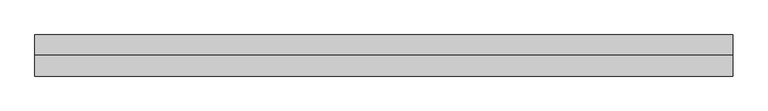
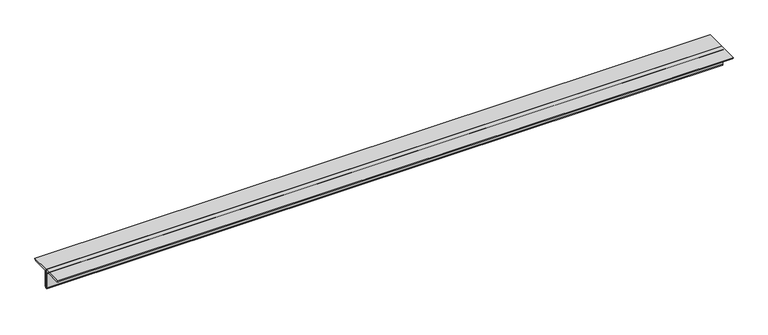
"""IFC4 building model written with IfcOpenShell, lengths in millimetres: member geometry, 0123_Steel Framing_2Ls-KSD3502 : H_SB_AR_S03_2Ls-130x130x12_HBR1."""

from ifc_helpers import new_model, si_unit, point, frame, frame_2d, origin, place, context, project, spatial, polyline, circle_curve, trimmed, segment, composite_curve, outline, extrude, source, transform, mapped, element, save


def member_7318b5d7(model_context):
    return source(origin(), model_context, "Body", "SweptSolid", [
        extrude(outline(composite_curve([segment(polyline([(0.0, 36.4), (0.0, -93.6)]), True, "CONTINUOUS"), segment(trimmed(circle_curve(frame_2d((0.0, -81.6)), 12.0), [point((0.0, -93.6))], [point((-12.0, -81.6))], False, "CARTESIAN"), True, "CONTINUOUS"), segment(polyline([(-12.0, -81.6), (-12.0, 12.4)]), True, "CONTINUOUS"), segment(trimmed(circle_curve(frame_2d((-24.0, 12.4)), 12.0), [point((-12.0, 12.4))], [point((-24.0, 24.4))], True, "CARTESIAN"), True, "CONTINUOUS"), segment(polyline([(-24.0, 24.4), (-118.0, 24.4)]), True, "CONTINUOUS"), segment(trimmed(circle_curve(frame_2d((-118.0, 36.4)), 12.0), [point((-118.0, 24.4))], [point((-130.0, 36.4))], False, "CARTESIAN"), True, "CONTINUOUS"), segment(polyline([(-130.0, 36.4), (0.0, 36.4)]), True, "CONTINUOUS")], self_intersect=False)), frame((-2254.4342987, 0.0, 0.0), z_axis=(1.0, 0.0, 0.0), x_axis=(0.0, 1.0, 0.0)), (0.0, 0.0, 1.0), 4412.2019305),
        extrude(outline(composite_curve([segment(polyline([(0.0, 36.4), (130.0, 36.4)]), True, "CONTINUOUS"), segment(trimmed(circle_curve(frame_2d((118.0, 36.4)), 12.0), [point((130.0, 36.4))], [point((118.0, 24.4))], False, "CARTESIAN"), True, "CONTINUOUS"), segment(polyline([(118.0, 24.4), (24.0, 24.4)]), True, "CONTINUOUS"), segment(trimmed(circle_curve(frame_2d((24.0, 12.4)), 12.0), [point((24.0, 24.4))], [point((12.0, 12.4))], True, "CARTESIAN"), True, "CONTINUOUS"), segment(polyline([(12.0, 12.4), (12.0, -81.6)]), True, "CONTINUOUS"), segment(trimmed(circle_curve(frame_2d((0.0, -81.6)), 12.0), [point((12.0, -81.6))], [point((0.0, -93.6))], False, "CARTESIAN"), True, "CONTINUOUS"), segment(polyline([(0.0, -93.6), (0.0, 36.4)]), True, "CONTINUOUS")], self_intersect=False)), frame((-2254.4342987, 0.0, 0.0), z_axis=(1.0, 0.0, 0.0), x_axis=(0.0, 1.0, 0.0)), (0.0, 0.0, 1.0), 4412.2019305),
    ])


if __name__ == "__main__":
    model = new_model("IFC4")
    model_context = context("Model", 3, world=origin())
    ifc_project = project(units=[si_unit("LENGTHUNIT", "METRE", prefix="MILLI")], contexts=[model_context])
    site = spatial("IfcSite", under=ifc_project)
    building = spatial("IfcBuilding", under=site)
    placement = place(None, origin())
    member_shape = member_7318b5d7(model_context)
    element("IfcMember", 1, ObjectType="0123_Steel Framing_2Ls-KSD3502 : H_SB_AR_S03_2Ls-130x130x12_HBR1", at=placement, inside=building, context=model_context, shape_type="MappedRepresentation", body=[
        mapped(member_shape, transform((0.0, 0.0, 0.0), x_axis=(1.0, 0.0, 0.0), y_axis=(0.0, 1.0, 0.0), z_axis=(0.0, 0.0, 1.0))),
    ])
    save(model, "model.ifc")

# Revit data of these elements
# Type "0123_Steel Framing_2Ls-KSD3502 : H_SB_AR_S03_2Ls-130x130x12_HBR1"
#   Type Mark = "HBR1"
#   Assembly Code = "B10"
#   Legs = "SLBB"
#   W = 8.97
#   Perimeter = 1.04 m²/m
#   Nominal Weight = 46.80 kgf/m
#   Length [instance default] = 1000 mm
#   Space = 0 mm
#   b = 130 mm
#   d = 130 mm
#   t = 12 mm
#   y = 36.4 mm
#   A = 0.005952 m²
#   Structural Material [instance default] = Steel ASTM A36
# Element 1 (IfcMember, "0123_Steel Framing_2Ls-KSD3502 : H_SB_AR_S03_2Ls-130x130x12_HBR1")
#   Materials on its faces: "Steel ASTM A36"
# Materials
#   "Steel ASTM A36": class "Metal", colour RGB 199 199 199, transparency 0, Description = "Structural steel, ASTM A36 Grade B, mill finish", Cost = 0
